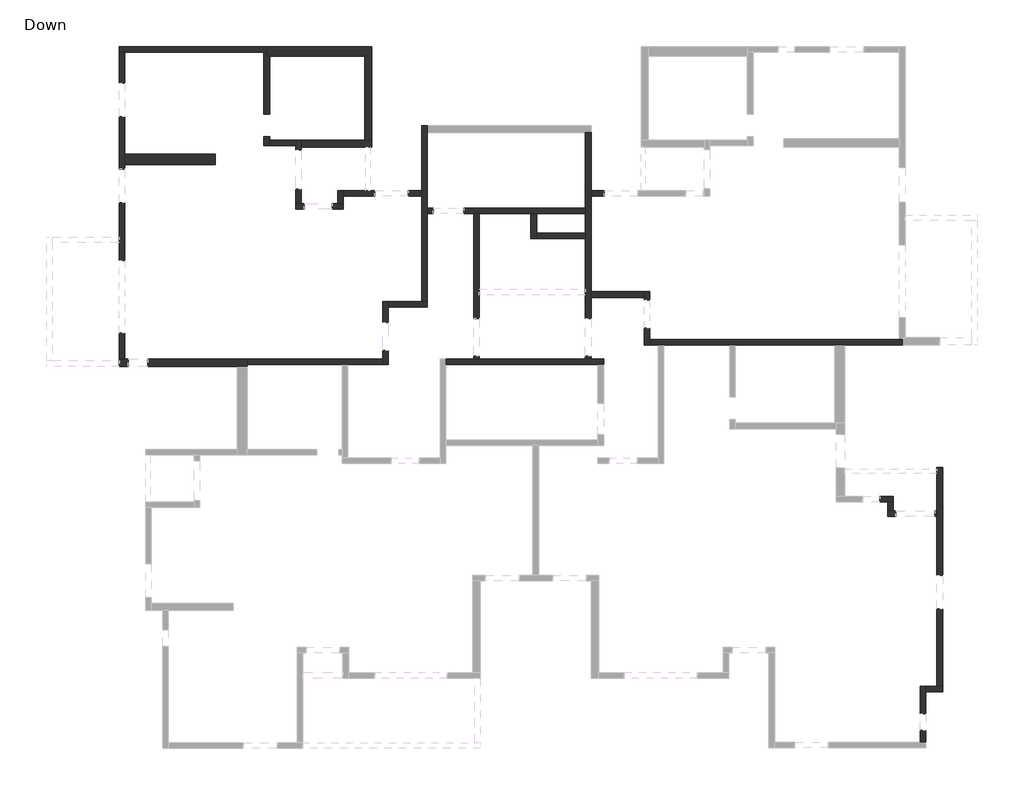
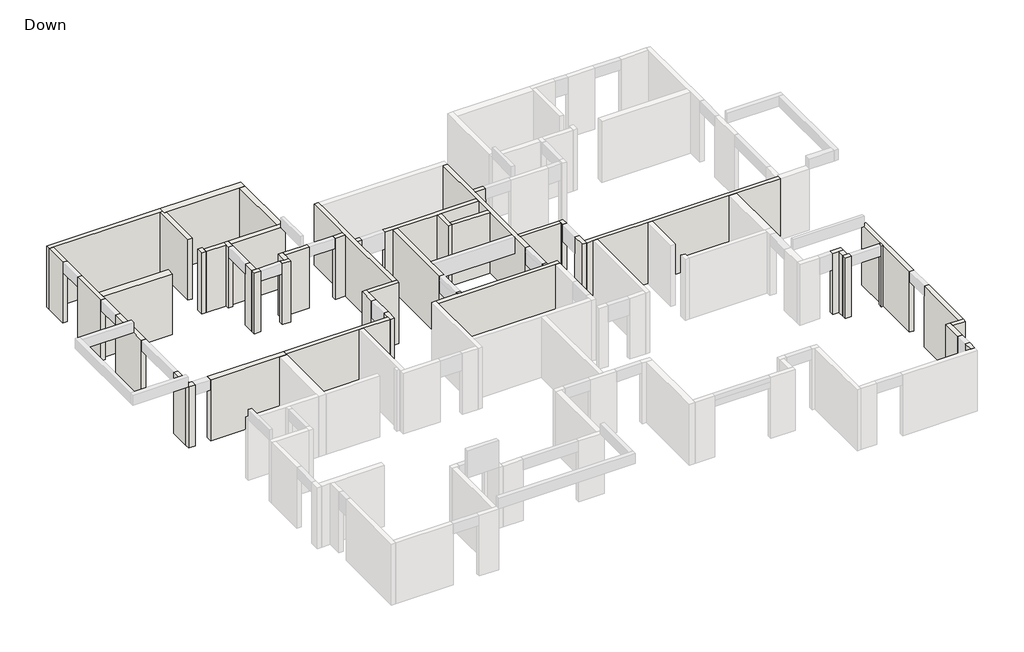
# One storey, part 2 of 3: 49 walls.
"""IFC4 building model written with IfcOpenShell, lengths in millimetres."""

from ifc_helpers import new_model, si_unit, origin, origin_with_axes, place, context, project, spatial, polyline, outline, extrude, faceted_brep, element, save

model = new_model("IFC4")

# Units and contexts
model_context = context("Model", 3, world=origin())
ifc_project = project(units=[si_unit("LENGTHUNIT", "METRE", prefix="MILLI")], contexts=[model_context])

# Site, building, storey
site = spatial("IfcSite", under=ifc_project)
building = spatial("IfcBuilding", under=site)
storey = spatial("IfcBuildingStorey", under=building, Name="Down", Elevation=0.0)

# Walls
placement = place(None, origin())
element("IfcWall", 1, ObjectType="20", at=placement, inside=storey, context=model_context, shape_type="Brep", body=[
    faceted_brep([(-5039.8370837, 11436.5624033, 0.0), (-10319.6462524, 11436.5624033, 0.0), (-10319.6462524, 11436.5624033, 3000.0), (-5039.8370837, 11436.5624033, 3000.0), (-5039.8370837, 11236.5624033, 0.0), (-5039.8370837, 11236.5624033, 3000.0), (-5139.8370837, 11236.5624033, 3000.0), (-10119.6462524, 11236.5624033, 3000.0), (-10319.6462524, 11236.5624033, 3000.0), (-10319.6462524, 11236.5624033, 0.0), (-10119.6462524, 11236.5624033, 0.0), (-5139.8370837, 11236.5624033, 0.0)], [[[0, 1, 2, 3]], [[4, 5, 6, 7, 8, 9, 10, 11]], [[1, 0, 4, 11, 10, 9]], [[3, 2, 8, 7, 6, 5]], [[0, 3, 5, 4]], [[2, 1, 9, 8]]]),
])
element("IfcWall", 2, ObjectType="20", at=placement, inside=storey, context=model_context, shape_type="Brep", body=[
    faceted_brep([(-10319.6462524, 11236.5624033, 0.0), (-10319.6462524, 10130.5632806, 0.0), (-10319.6462524, 10130.5632806, 2500.0), (-10319.6462524, 10130.5632806, 3000.0), (-10319.6462524, 11236.5624033, 3000.0), (-10119.6462524, 11236.5624033, 0.0), (-10119.6462524, 11236.5624033, 2780.0), (-10119.6462524, 11236.5624033, 3000.0), (-10119.6462524, 10130.5632806, 3000.0), (-10119.6462524, 10130.5632806, 2500.0), (-10119.6462524, 10130.5632806, 0.0)], [[[0, 1, 2, 3, 4]], [[5, 6, 7, 8, 9, 10]], [[1, 0, 5, 10]], [[3, 2, 1, 10, 9, 8]], [[4, 3, 8, 7]], [[0, 4, 7, 6, 5]]]),
])
element("IfcWall", 3, ObjectType="20", at=placement, inside=storey, context=model_context, shape_type="Brep", body=[
    faceted_brep([(-10319.6462524, 8930.3987709, 0.0), (-10319.6462524, 7055.0094311, 0.0), (-10319.6462524, 7055.0094311, 2500.0), (-10319.6462524, 7055.0094311, 3000.0), (-10319.6462524, 8930.3987709, 3000.0), (-10319.6462524, 8930.3987709, 2500.0), (-10119.6462524, 8930.3987709, 0.0), (-10119.6462524, 8930.3987709, 2500.0), (-10119.6462524, 8930.3987709, 3000.0), (-10119.6462524, 7575.1187953, 3000.0), (-10119.6462524, 7215.1187953, 3000.0), (-10119.6462524, 7055.0094311, 3000.0), (-10119.6462524, 7055.0094311, 2500.0), (-10119.6462524, 7055.0094311, 0.0), (-10119.6462524, 7215.1187953, 0.0), (-10119.6462524, 7575.1187953, 0.0)], [[[0, 1, 2, 3, 4, 5]], [[6, 7, 8, 9, 10, 11, 12, 13, 14, 15]], [[1, 0, 6, 15, 14, 13]], [[3, 2, 1, 13, 12, 11]], [[4, 3, 11, 10, 9, 8]], [[0, 5, 4, 8, 7, 6]]]),
])
element("IfcWall", 4, ObjectType="20", at=placement, inside=storey, context=model_context, shape_type="Brep", body=[
    faceted_brep([(-10319.6462524, 5854.8449214, 0.0), (-10319.6462524, 3780.4865094, 0.0), (-10319.6462524, 3780.4865094, 2500.0), (-10319.6462524, 3780.4865094, 3000.0), (-10319.6462524, 4616.1884177, 3000.0), (-10319.6462524, 5854.8449214, 3000.0), (-10319.6462524, 5854.8449214, 2500.0), (-10119.6462524, 5854.8449214, 0.0), (-10119.6462524, 5854.8449214, 2500.0), (-10119.6462524, 5854.8449214, 3000.0), (-10119.6462524, 3780.4865094, 3000.0), (-10119.6462524, 3780.4865094, 2500.0), (-10119.6462524, 3780.4865094, 0.0)], [[[0, 1, 2, 3, 4, 5, 6]], [[7, 8, 9, 10, 11, 12]], [[1, 0, 7, 12]], [[3, 2, 1, 12, 11, 10]], [[5, 4, 3, 10, 9]], [[0, 6, 5, 9, 8, 7]]]),
])
element("IfcWall", 5, ObjectType="20", at=placement, inside=storey, context=model_context, shape_type="Brep", body=[
    faceted_brep([(-10319.6462524, 1181.1884177, 0.0), (-10319.6462524, 251.1884177, 0.0), (-10319.6462524, 251.1884177, 3000.0), (-10319.6462524, 1181.1884177, 3000.0), (-10319.6462524, 1181.1884177, 2500.0), (-10119.6462524, 1181.1884177, 0.0), (-10119.6462524, 1181.1884177, 2500.0), (-10119.6462524, 1181.1884177, 3000.0), (-10119.6462524, 251.1884177, 3000.0), (-10119.6462524, 251.1884177, 2780.0), (-10119.6462524, 251.1884177, 0.0)], [[[0, 1, 2, 3, 4]], [[5, 6, 7, 8, 9, 10]], [[1, 0, 5, 10]], [[3, 2, 8, 7]], [[0, 4, 3, 7, 6, 5]], [[2, 1, 10, 9, 8]]]),
])
element("IfcWall", 6, ObjectType="20", at=placement, inside=storey, context=model_context, shape_type="Brep", body=[
    faceted_brep([(-5740.9338154, 51.1884177, 0.0), (-2336.5139865, 51.1884177, 0.0), (-2136.5139865, 51.1884177, 0.0), (-890.8131749, 51.1884177, 0.0), (-890.8131749, 51.1884177, 3000.0), (-2136.5139865, 51.1884177, 3000.0), (-2336.5139865, 51.1884177, 3000.0), (-5740.9338154, 51.1884177, 3000.0), (-5740.9338154, 51.1884177, 2780.0), (-5740.9338154, 251.1884177, 0.0), (-5740.9338154, 251.1884177, 3000.0), (-890.8131749, 251.1884177, 3000.0), (-890.8131749, 251.1884177, 2780.0), (-890.8131749, 251.1884177, 0.0)], [[[0, 1, 2, 3, 4, 5, 6, 7, 8]], [[9, 10, 11, 12, 13]], [[3, 2, 1, 0, 9, 13]], [[7, 6, 5, 4, 11, 10]], [[0, 8, 7, 10, 9]], [[4, 3, 13, 12, 11]]]),
])
element("IfcWall", 7, ObjectType="20", at=placement, inside=storey, context=model_context, shape_type="Brep", body=[
    faceted_brep([(-690.8131749, 51.1884177, 0.0), (-690.8131749, 556.7642019, 0.0), (-690.8131749, 556.7642019, 2180.0), (-690.8131749, 556.7642019, 3000.0), (-690.8131749, 51.1884177, 3000.0), (-690.8131749, 51.1884177, 2780.0), (-890.8131749, 51.1884177, 0.0), (-890.8131749, 51.1884177, 3000.0), (-890.8131749, 251.1884177, 3000.0), (-890.8131749, 556.7642019, 3000.0), (-890.8131749, 556.7642019, 2180.0), (-890.8131749, 556.7642019, 0.0), (-890.8131749, 251.1884177, 0.0)], [[[0, 1, 2, 3, 4, 5]], [[6, 7, 8, 9, 10, 11, 12]], [[1, 0, 6, 12, 11]], [[3, 2, 1, 11, 10, 9]], [[4, 3, 9, 8, 7]], [[0, 5, 4, 7, 6]]]),
])
element("IfcWall", 8, ObjectType="20", at=placement, inside=storey, context=model_context, shape_type="Brep", body=[
    faceted_brep([(-690.8131749, 1555.8429472, 0.0), (-690.8131749, 2105.1520062, 0.0), (-690.8131749, 2305.1520062, 0.0), (-690.8131749, 2305.1520062, 3000.0), (-690.8131749, 2105.1520062, 3000.0), (-690.8131749, 1555.8429472, 3000.0), (-690.8131749, 1555.8429472, 2180.0), (-890.8131749, 1555.8429472, 0.0), (-890.8131749, 1555.8429472, 2180.0), (-890.8131749, 1555.8429472, 3000.0), (-890.8131749, 2305.1520062, 3000.0), (-890.8131749, 2305.1520062, 2780.0), (-890.8131749, 2305.1520062, 0.0)], [[[0, 1, 2, 3, 4, 5, 6]], [[7, 8, 9, 10, 11, 12]], [[2, 1, 0, 7, 12]], [[5, 4, 3, 10, 9]], [[0, 6, 5, 9, 8, 7]], [[3, 2, 12, 11, 10]]]),
])
element("IfcWall", 9, ObjectType="20", at=placement, inside=storey, context=model_context, shape_type="Brep", body=[
    faceted_brep([(-690.8131749, 2105.1520062, 0.0), (708.320407, 2105.1520062, 0.0), (708.320407, 2105.1520062, 2780.0), (708.320407, 2105.1520062, 3000.0), (-690.8131749, 2105.1520062, 3000.0), (-690.8131749, 2105.1520062, 2780.0), (-690.8131749, 2305.1520062, 0.0), (-690.8131749, 2305.1520062, 3000.0), (508.320407, 2305.1520062, 3000.0), (708.320407, 2305.1520062, 3000.0), (708.320407, 2305.1520062, 0.0), (508.320407, 2305.1520062, 0.0)], [[[0, 1, 2, 3, 4, 5]], [[6, 7, 8, 9, 10, 11]], [[1, 0, 6, 11, 10]], [[4, 3, 9, 8, 7]], [[0, 5, 4, 7, 6]], [[3, 2, 1, 10, 9]]]),
])
element("IfcWall", 10, ObjectType="20", at=placement, inside=storey, context=model_context, shape_type="Brep", body=[
    faceted_brep([(708.320407, 2305.1520062, 0.0), (708.320407, 5455.8758492, 0.0), (708.320407, 5655.8758492, 0.0), (708.320407, 8355.1520062, 0.0), (708.320407, 8605.1520062, 0.0), (708.320407, 8605.1520062, 3000.0), (708.320407, 8355.1520062, 3000.0), (708.320407, 5655.8758492, 3000.0), (708.320407, 5455.8758492, 3000.0), (708.320407, 2305.1520062, 3000.0), (508.320407, 2305.1520062, 0.0), (508.320407, 2305.1520062, 2780.0), (508.320407, 2305.1520062, 3000.0), (508.320407, 6080.1520062, 3000.0), (508.320407, 6280.1520062, 3000.0), (508.320407, 8605.1520062, 3000.0), (508.320407, 8605.1520062, 0.0), (508.320407, 6280.1520062, 0.0), (508.320407, 6080.1520062, 0.0)], [[[0, 1, 2, 3, 4, 5, 6, 7, 8, 9]], [[10, 11, 12, 13, 14, 15, 16, 17, 18]], [[4, 3, 2, 1, 0, 10, 18, 17, 16]], [[9, 8, 7, 6, 5, 15, 14, 13, 12]], [[0, 9, 12, 11, 10]], [[5, 4, 16, 15]]]),
])
element("IfcWall", 11, ObjectType="20", at=placement, inside=storey, context=model_context, shape_type="Brep", body=[
    faceted_brep([(708.320407, 5455.8758492, 0.0), (909.4061714, 5455.8758492, 0.0), (909.4061714, 5455.8758492, 2180.0), (909.4061714, 5455.8758492, 3000.0), (708.320407, 5455.8758492, 3000.0), (708.320407, 5455.8758492, 2780.0), (708.320407, 5655.8758492, 0.0), (708.320407, 5655.8758492, 2780.0), (708.320407, 5655.8758492, 3000.0), (909.4061714, 5655.8758492, 3000.0), (909.4061714, 5655.8758492, 2180.0), (909.4061714, 5655.8758492, 0.0)], [[[0, 1, 2, 3, 4, 5]], [[6, 7, 8, 9, 10, 11]], [[1, 0, 6, 11]], [[3, 2, 1, 11, 10, 9]], [[4, 3, 9, 8]], [[0, 5, 4, 8, 7, 6]]]),
])
element("IfcWall", 12, ObjectType="20", at=placement, inside=storey, context=model_context, shape_type="Brep", body=[
    faceted_brep([(508.320407, 6280.1520062, 0.0), (28.320407, 6280.1520062, 0.0), (28.320407, 6280.1520062, 2500.0), (28.320407, 6280.1520062, 3000.0), (508.320407, 6280.1520062, 3000.0), (508.320407, 6080.1520062, 0.0), (508.320407, 6080.1520062, 2780.0), (508.320407, 6080.1520062, 3000.0), (28.320407, 6080.1520062, 3000.0), (28.320407, 6080.1520062, 2500.0), (28.320407, 6080.1520062, 0.0)], [[[0, 1, 2, 3, 4]], [[5, 6, 7, 8, 9, 10]], [[1, 0, 5, 10]], [[3, 2, 1, 10, 9, 8]], [[4, 3, 8, 7]], [[0, 4, 7, 6, 5]]]),
])
element("IfcWall", 13, ObjectType="20", at=placement, inside=storey, context=model_context, shape_type="Brep", body=[
    faceted_brep([(-1171.679593, 6280.1520062, 0.0), (-2301.679593, 6280.1520062, 0.0), (-2301.679593, 6280.1520062, 3000.0), (-1339.8370837, 6280.1520062, 3000.0), (-1171.679593, 6280.1520062, 3000.0), (-1171.679593, 6280.1520062, 2500.0), (-1171.679593, 6080.1520062, 0.0), (-1171.679593, 6080.1520062, 2500.0), (-1171.679593, 6080.1520062, 3000.0), (-2301.679593, 6080.1520062, 3000.0), (-2301.679593, 6080.1520062, 2780.0), (-2301.679593, 6080.1520062, 0.0)], [[[0, 1, 2, 3, 4, 5]], [[6, 7, 8, 9, 10, 11]], [[1, 0, 6, 11]], [[4, 3, 2, 9, 8]], [[0, 5, 4, 8, 7, 6]], [[2, 1, 11, 10, 9]]]),
])
element("IfcWall", 14, ObjectType="20", at=placement, inside=storey, context=model_context, shape_type="Brep", body=[
    faceted_brep([(-2501.679593, 6280.1520062, 0.0), (-2501.679593, 5815.1520062, 0.0), (-2501.679593, 5815.1520062, 2780.0), (-2501.679593, 5815.1520062, 3000.0), (-2501.679593, 6280.1520062, 3000.0), (-2501.679593, 6280.1520062, 2780.0), (-2301.679593, 6280.1520062, 0.0), (-2301.679593, 6280.1520062, 3000.0), (-2301.679593, 6080.1520062, 3000.0), (-2301.679593, 5815.1520062, 3000.0), (-2301.679593, 5815.1520062, 0.0), (-2301.679593, 6080.1520062, 0.0)], [[[0, 1, 2, 3, 4, 5]], [[6, 7, 8, 9, 10, 11]], [[1, 0, 6, 11, 10]], [[4, 3, 9, 8, 7]], [[0, 5, 4, 7, 6]], [[3, 2, 1, 10, 9]]]),
])
element("IfcWall", 15, ObjectType="20", at=placement, inside=storey, context=model_context, shape_type="Brep", body=[
    faceted_brep([(-2301.679593, 5815.1520062, 0.0), (-2501.679593, 5815.1520062, 0.0), (-2696.679593, 5815.1520062, 0.0), (-2696.679593, 5815.1520062, 2500.0), (-2696.679593, 5815.1520062, 3000.0), (-2501.679593, 5815.1520062, 3000.0), (-2301.679593, 5815.1520062, 3000.0), (-2301.679593, 5615.1520062, 0.0), (-2301.679593, 5615.1520062, 2780.0), (-2301.679593, 5615.1520062, 3000.0), (-2696.679593, 5615.1520062, 3000.0), (-2696.679593, 5615.1520062, 2500.0), (-2696.679593, 5615.1520062, 0.0)], [[[0, 1, 2, 3, 4, 5, 6]], [[7, 8, 9, 10, 11, 12]], [[2, 1, 0, 7, 12]], [[4, 3, 2, 12, 11, 10]], [[6, 5, 4, 10, 9]], [[0, 6, 9, 8, 7]]]),
])
element("IfcWall", 16, ObjectType="20", at=placement, inside=storey, context=model_context, shape_type="Brep", body=[
    faceted_brep([(-3696.679593, 5815.1520062, 0.0), (-3799.8370837, 5815.1520062, 0.0), (-3999.8370837, 5815.1520062, 0.0), (-3999.8370837, 5815.1520062, 3000.0), (-3799.8370837, 5815.1520062, 3000.0), (-3696.679593, 5815.1520062, 3000.0), (-3696.679593, 5815.1520062, 2500.0), (-3696.679593, 5615.1520062, 0.0), (-3696.679593, 5615.1520062, 2500.0), (-3696.679593, 5615.1520062, 3000.0), (-3999.8370837, 5615.1520062, 3000.0), (-3999.8370837, 5615.1520062, 2780.0), (-3999.8370837, 5615.1520062, 0.0)], [[[0, 1, 2, 3, 4, 5, 6]], [[7, 8, 9, 10, 11, 12]], [[2, 1, 0, 7, 12]], [[5, 4, 3, 10, 9]], [[0, 6, 5, 9, 8, 7]], [[3, 2, 12, 11, 10]]]),
])
element("IfcWall", 17, ObjectType="20", at=placement, inside=storey, context=model_context, shape_type="Brep", body=[
    faceted_brep([(-3799.8370837, 5815.1520062, 0.0), (-3799.8370837, 6335.1520062, 0.0), (-3799.8370837, 6335.1520062, 2500.0), (-3799.8370837, 6335.1520062, 3000.0), (-3799.8370837, 5815.1520062, 3000.0), (-3799.8370837, 5815.1520062, 2780.0), (-3999.8370837, 5815.1520062, 0.0), (-3999.8370837, 5815.1520062, 3000.0), (-3999.8370837, 6335.1520062, 3000.0), (-3999.8370837, 6335.1520062, 2500.0), (-3999.8370837, 6335.1520062, 0.0)], [[[0, 1, 2, 3, 4, 5]], [[6, 7, 8, 9, 10]], [[1, 0, 6, 10]], [[3, 2, 1, 10, 9, 8]], [[4, 3, 8, 7]], [[0, 5, 4, 7, 6]]]),
])
element("IfcWall", 18, ObjectType="20", at=placement, inside=storey, context=model_context, shape_type="Brep", body=[
    faceted_brep([(-5139.8370837, 11236.5624033, 0.0), (-5139.8370837, 9006.5624033, 0.0), (-5139.8370837, 9006.5624033, 2780.0), (-5139.8370837, 9006.5624033, 3000.0), (-5139.8370837, 11236.5624033, 3000.0), (-5139.8370837, 11236.5624033, 2780.0), (-4939.8370837, 11086.5624033, 0.0), (-4939.8370837, 11086.5624033, 2780.0), (-4939.8370837, 11086.5624033, 3000.0), (-4939.8370837, 9006.5624033, 3000.0), (-4939.8370837, 9006.5624033, 2780.0), (-4939.8370837, 9006.5624033, 0.0), (-5039.8370837, 11236.5624033, 0.0), (-5039.8370837, 11086.5624033, 0.0), (-5039.8370837, 11086.5624033, 3000.0), (-5039.8370837, 11236.5624033, 3000.0)], [[[0, 1, 2, 3, 4, 5]], [[6, 7, 8, 9, 10, 11]], [[1, 0, 12, 13, 6, 11]], [[3, 2, 1, 11, 10, 9]], [[4, 3, 9, 8, 14, 15]], [[0, 5, 4, 15, 12]], [[15, 14, 13, 12]], [[14, 8, 7, 6, 13]]]),
])
element("IfcWall", 19, ObjectType="20", at=placement, inside=storey, context=model_context, shape_type="Brep", body=[
    faceted_brep([(-5139.8370837, 8206.5624033, 0.0), (-5139.8370837, 7886.5624033, 0.0), (-5139.8370837, 7886.5624033, 2780.0), (-5139.8370837, 7886.5624033, 3000.0), (-5139.8370837, 8206.5624033, 3000.0), (-5139.8370837, 8206.5624033, 2780.0), (-4939.8370837, 8206.5624033, 0.0), (-4939.8370837, 8206.5624033, 2780.0), (-4939.8370837, 8206.5624033, 3000.0), (-4939.8370837, 8086.5624033, 3000.0), (-4939.8370837, 7886.5624033, 3000.0), (-4939.8370837, 7886.5624033, 0.0), (-4939.8370837, 8086.5624033, 0.0)], [[[0, 1, 2, 3, 4, 5]], [[6, 7, 8, 9, 10, 11, 12]], [[1, 0, 6, 12, 11]], [[4, 3, 10, 9, 8]], [[0, 5, 4, 8, 7, 6]], [[3, 2, 1, 11, 10]]]),
])
element("IfcWall", 20, ObjectType="20", at=placement, inside=storey, context=model_context, shape_type="Brep", body=[
    faceted_brep([(-4939.8370837, 7886.5624033, 0.0), (-3999.8370837, 7886.5624033, 0.0), (-3999.8370837, 7886.5624033, 2780.0), (-3999.8370837, 7886.5624033, 3000.0), (-4939.8370837, 7886.5624033, 3000.0), (-4939.8370837, 8086.5624033, 0.0), (-4939.8370837, 8086.5624033, 2780.0), (-4939.8370837, 8086.5624033, 3000.0), (-3999.8370837, 8086.5624033, 3000.0), (-3999.8370837, 8086.5624033, 0.0)], [[[0, 1, 2, 3, 4]], [[5, 6, 7, 8, 9]], [[1, 0, 5, 9]], [[4, 3, 8, 7]], [[0, 4, 7, 6, 5]], [[3, 2, 1, 9, 8]]]),
])
element("IfcWall", 21, ObjectType="20", at=placement, inside=storey, context=model_context, shape_type="Brep", body=[
    faceted_brep([(-3999.8370837, 8086.5624033, 0.0), (-3999.8370837, 7886.5624033, 0.0), (-3999.8370837, 7726.5624033, 0.0), (-3999.8370837, 7726.5624033, 2500.0), (-3999.8370837, 7726.5624033, 3000.0), (-3999.8370837, 7886.5624033, 3000.0), (-3999.8370837, 8086.5624033, 3000.0), (-3799.8370837, 8086.5624033, 0.0), (-3799.8370837, 8086.5624033, 3000.0), (-3799.8370837, 7836.5624033, 3000.0), (-3799.8370837, 7726.5624033, 3000.0), (-3799.8370837, 7726.5624033, 2500.0), (-3799.8370837, 7726.5624033, 0.0), (-3799.8370837, 7836.5624033, 0.0)], [[[0, 1, 2, 3, 4, 5, 6]], [[7, 8, 9, 10, 11, 12, 13]], [[2, 1, 0, 7, 13, 12]], [[4, 3, 2, 12, 11, 10]], [[6, 5, 4, 10, 9, 8]], [[0, 6, 8, 7]]]),
])
element("IfcWall", 22, ObjectType="20", at=placement, inside=storey, context=model_context, shape_type="Brep", body=[
    faceted_brep([(6363.320407, 8355.1520062, 0.0), (6363.320407, 5655.8758492, 0.0), (6363.320407, 5455.8758492, 0.0), (6363.320407, 4755.8758492, 0.0), (6363.320407, 4555.8758492, 0.0), (6363.320407, 1705.1520062, 0.0), (6363.320407, 1705.1520062, 2180.0), (6363.320407, 1705.1520062, 2780.0), (6363.320407, 1705.1520062, 3000.0), (6363.320407, 2545.8758492, 3000.0), (6363.320407, 2745.8758492, 3000.0), (6363.320407, 4555.8758492, 3000.0), (6363.320407, 4755.8758492, 3000.0), (6363.320407, 5455.8758492, 3000.0), (6363.320407, 5655.8758492, 3000.0), (6363.320407, 8355.1520062, 3000.0), (6563.320407, 8355.1520062, 0.0), (6563.320407, 8355.1520062, 3000.0), (6563.320407, 6284.3445962, 3000.0), (6563.320407, 6084.3445962, 3000.0), (6563.320407, 2655.1520062, 3000.0), (6563.320407, 2455.1520062, 3000.0), (6563.320407, 1705.1520062, 3000.0), (6563.320407, 1705.1520062, 2180.0), (6563.320407, 1705.1520062, 0.0), (6563.320407, 2455.1520062, 0.0), (6563.320407, 2655.1520062, 0.0), (6563.320407, 6084.3445962, 0.0), (6563.320407, 6284.3445962, 0.0), (6368.320407, 1705.1520062, 3000.0)], [[[0, 1, 2, 3, 4, 5, 6, 7, 8, 9, 10, 11, 12, 13, 14, 15]], [[16, 17, 18, 19, 20, 21, 22, 23, 24, 25, 26, 27, 28]], [[5, 4, 3, 2, 1, 0, 16, 28, 27, 26, 25, 24]], [[8, 7, 6, 5, 24, 23, 22, 29]], [[15, 14, 13, 12, 11, 10, 9, 8, 29, 22, 21, 20, 19, 18, 17]], [[0, 15, 17, 16]]]),
])
element("IfcWall", 23, ObjectType="20", at=placement, inside=storey, context=model_context, shape_type="Brep", body=[
    faceted_brep([(6563.320407, 2455.1520062, 0.0), (8463.320407, 2455.1520062, 0.0), (8463.320407, 2455.1520062, 2780.0), (8463.320407, 2455.1520062, 3000.0), (6563.320407, 2455.1520062, 3000.0), (6563.320407, 2455.1520062, 2780.0), (6563.320407, 2655.1520062, 0.0), (6563.320407, 2655.1520062, 2780.0), (6563.320407, 2655.1520062, 3000.0), (8463.320407, 2655.1520062, 3000.0), (8463.320407, 2655.1520062, 0.0)], [[[0, 1, 2, 3, 4, 5]], [[6, 7, 8, 9, 10]], [[1, 0, 6, 10]], [[4, 3, 9, 8]], [[0, 5, 4, 8, 7, 6]], [[3, 2, 1, 10, 9]]]),
])
element("IfcWall", 24, ObjectType="20", at=placement, inside=storey, context=model_context, shape_type="Brep", body=[
    faceted_brep([(8463.320407, 2655.1520062, 0.0), (8463.320407, 2455.1520062, 0.0), (8463.320407, 2355.1520062, 0.0), (8463.320407, 2355.1520062, 2180.0), (8463.320407, 2355.1520062, 3000.0), (8463.320407, 2455.1520062, 3000.0), (8463.320407, 2655.1520062, 3000.0), (8663.320407, 2655.1520062, 0.0), (8663.320407, 2655.1520062, 2780.0), (8663.320407, 2655.1520062, 3000.0), (8663.320407, 2355.1520062, 3000.0), (8663.320407, 2355.1520062, 2180.0), (8663.320407, 2355.1520062, 0.0)], [[[0, 1, 2, 3, 4, 5, 6]], [[7, 8, 9, 10, 11, 12]], [[2, 1, 0, 7, 12]], [[4, 3, 2, 12, 11, 10]], [[6, 5, 4, 10, 9]], [[0, 6, 9, 8, 7]]]),
])
element("IfcWall", 25, ObjectType="20", at=placement, inside=storey, context=model_context, shape_type="Brep", body=[
    faceted_brep([(6363.320407, 5655.8758492, 0.0), (2013.320407, 5655.8758492, 0.0), (2013.320407, 5655.8758492, 2180.0), (2013.320407, 5655.8758492, 3000.0), (2460.820407, 5655.8758492, 3000.0), (6363.320407, 5655.8758492, 3000.0), (6363.320407, 5455.8758492, 0.0), (6363.320407, 5455.8758492, 3000.0), (4613.320407, 5455.8758492, 3000.0), (4413.320407, 5455.8758492, 3000.0), (2560.820407, 5455.8758492, 3000.0), (2360.820407, 5455.8758492, 3000.0), (2013.320407, 5455.8758492, 3000.0), (2013.320407, 5455.8758492, 2180.0), (2013.320407, 5455.8758492, 0.0), (2360.820407, 5455.8758492, 0.0), (2560.820407, 5455.8758492, 0.0), (4413.320407, 5455.8758492, 0.0), (4613.320407, 5455.8758492, 0.0)], [[[0, 1, 2, 3, 4, 5]], [[6, 7, 8, 9, 10, 11, 12, 13, 14, 15, 16, 17, 18]], [[1, 0, 6, 18, 17, 16, 15, 14]], [[3, 2, 1, 14, 13, 12]], [[5, 4, 3, 12, 11, 10, 9, 8, 7]], [[0, 5, 7, 6]]]),
])
element("IfcWall", 26, ObjectType="20", at=placement, inside=storey, context=model_context, shape_type="Brep", body=[
    faceted_brep([(2360.820407, 5455.8758492, 0.0), (2360.820407, 1705.8758492, 0.0), (2360.820407, 1705.8758492, 2180.0), (2360.820407, 1705.8758492, 2780.0), (2360.820407, 1705.8758492, 3000.0), (2360.820407, 5455.8758492, 3000.0), (2360.820407, 5455.8758492, 2780.0), (2560.820407, 5455.8758492, 0.0), (2560.820407, 5455.8758492, 3000.0), (2560.820407, 2745.8758492, 3000.0), (2560.820407, 2545.8758492, 3000.0), (2560.820407, 1705.8758492, 3000.0), (2560.820407, 1705.8758492, 2180.0), (2560.820407, 1705.8758492, 0.0), (2363.3932055, 1705.8758492, 3000.0)], [[[0, 1, 2, 3, 4, 5, 6]], [[7, 8, 9, 10, 11, 12, 13]], [[1, 0, 7, 13]], [[4, 3, 2, 1, 13, 12, 11, 14]], [[5, 4, 14, 11, 10, 9, 8]], [[0, 6, 5, 8, 7]]]),
])
element("IfcWall", 27, ObjectType="20", at=placement, inside=storey, context=model_context, shape_type="Brep", body=[
    faceted_brep([(2360.820407, 352.3535615, 0.0), (2360.820407, 252.3535615, 0.0), (2360.820407, 252.3535615, 2780.0), (2360.820407, 252.3535615, 3000.0), (2360.820407, 352.3535615, 3000.0), (2360.820407, 352.3535615, 2780.0), (2360.820407, 352.3535615, 2180.0), (2560.820407, 352.3535615, 0.0), (2560.820407, 352.3535615, 2180.0), (2560.820407, 352.3535615, 3000.0), (2560.820407, 252.3535615, 3000.0), (2560.820407, 252.3535615, 0.0), (2363.3932055, 352.3535615, 3000.0)], [[[0, 1, 2, 3, 4, 5, 6]], [[7, 8, 9, 10, 11]], [[1, 0, 7, 11]], [[4, 3, 10, 9, 12]], [[0, 6, 5, 4, 12, 9, 8, 7]], [[3, 2, 1, 11, 10]]]),
])
element("IfcWall", 28, ObjectType="20", at=placement, inside=storey, context=model_context, shape_type="Brep", body=[
    faceted_brep([(1360.820407, 52.3535615, 0.0), (6810.820407, 52.3535615, 0.0), (7010.820407, 52.3535615, 0.0), (7010.820407, 52.3535615, 3000.0), (6810.820407, 52.3535615, 3000.0), (1360.820407, 52.3535615, 3000.0), (1360.820407, 252.3535615, 0.0), (1360.820407, 252.3535615, 3000.0), (2360.820407, 252.3535615, 3000.0), (2560.820407, 252.3535615, 3000.0), (6363.320407, 252.3535615, 3000.0), (6563.320407, 252.3535615, 3000.0), (7010.820407, 252.3535615, 3000.0), (7010.820407, 252.3535615, 2780.0), (7010.820407, 252.3535615, 0.0), (6563.320407, 252.3535615, 0.0), (6363.320407, 252.3535615, 0.0), (2560.820407, 252.3535615, 0.0), (2360.820407, 252.3535615, 0.0)], [[[0, 1, 2, 3, 4, 5]], [[6, 7, 8, 9, 10, 11, 12, 13, 14, 15, 16, 17, 18]], [[2, 1, 0, 6, 18, 17, 16, 15, 14]], [[5, 4, 3, 12, 11, 10, 9, 8, 7]], [[3, 2, 14, 13, 12]], [[0, 5, 7, 6]]]),
])
element("IfcWall", 29, ObjectType="20", at=placement, inside=storey, context=model_context, shape_type="Brep", body=[
    faceted_brep([(18537.905294, -13477.9835498, 0.0), (18537.905294, -13047.9835498, 0.0), (18537.905294, -13047.9835498, 2180.0), (18537.905294, -13047.9835498, 3000.0), (18537.905294, -13477.9835498, 3000.0), (18337.905294, -13477.9835498, 0.0), (18337.905294, -13477.9835498, 2780.0), (18337.905294, -13477.9835498, 3000.0), (18337.905294, -13047.9835498, 3000.0), (18337.905294, -13047.9835498, 2180.0), (18337.905294, -13047.9835498, 0.0)], [[[0, 1, 2, 3, 4]], [[5, 6, 7, 8, 9, 10]], [[1, 0, 5, 10]], [[3, 2, 1, 10, 9, 8]], [[4, 3, 8, 7]], [[0, 4, 7, 6, 5]]]),
])
element("IfcWall", 30, ObjectType="20", at=placement, inside=storey, context=model_context, shape_type="Brep", body=[
    faceted_brep([(18537.905294, -12447.9835498, 0.0), (18537.905294, -11672.9835498, 0.0), (18537.905294, -11472.9835498, 0.0), (18537.905294, -11472.9835498, 3000.0), (18537.905294, -11672.9835498, 3000.0), (18537.905294, -12447.9835498, 3000.0), (18537.905294, -12447.9835498, 2180.0), (18337.905294, -12447.9835498, 0.0), (18337.905294, -12447.9835498, 2180.0), (18337.905294, -12447.9835498, 3000.0), (18337.905294, -11472.9835498, 3000.0), (18337.905294, -11472.9835498, 2780.0), (18337.905294, -11472.9835498, 0.0)], [[[0, 1, 2, 3, 4, 5, 6]], [[7, 8, 9, 10, 11, 12]], [[2, 1, 0, 7, 12]], [[5, 4, 3, 10, 9]], [[0, 6, 5, 9, 8, 7]], [[3, 2, 12, 11, 10]]]),
])
element("IfcWall", 31, ObjectType="20", at=placement, inside=storey, context=model_context, shape_type="Brep", body=[
    faceted_brep([(18537.905294, -11672.9835498, 0.0), (19137.905294, -11672.9835498, 0.0), (19137.905294, -11672.9835498, 3000.0), (18537.905294, -11672.9835498, 3000.0), (18537.905294, -11472.9835498, 0.0), (18537.905294, -11472.9835498, 3000.0), (18937.905294, -11472.9835498, 3000.0), (19137.905294, -11472.9835498, 3000.0), (19137.905294, -11472.9835498, 0.0), (18937.905294, -11472.9835498, 0.0)], [[[0, 1, 2, 3]], [[4, 5, 6, 7, 8, 9]], [[1, 0, 4, 9, 8]], [[3, 2, 7, 6, 5]], [[0, 3, 5, 4]], [[2, 1, 8, 7]]]),
])
element("IfcWall", 32, ObjectType="20", at=placement, inside=storey, context=model_context, shape_type="Brep", body=[
    faceted_brep([(19137.905294, -11472.9835498, 0.0), (19137.905294, -8697.9835498, 0.0), (19137.905294, -8697.9835498, 2500.0), (19137.905294, -8697.9835498, 3000.0), (19137.905294, -11472.9835498, 3000.0), (18937.905294, -11472.9835498, 0.0), (18937.905294, -11472.9835498, 2780.0), (18937.905294, -11472.9835498, 3000.0), (18937.905294, -8697.9835498, 3000.0), (18937.905294, -8697.9835498, 2500.0), (18937.905294, -8697.9835498, 0.0)], [[[0, 1, 2, 3, 4]], [[5, 6, 7, 8, 9, 10]], [[1, 0, 5, 10]], [[3, 2, 1, 10, 9, 8]], [[4, 3, 8, 7]], [[0, 4, 7, 6, 5]]]),
])
element("IfcWall", 33, ObjectType="20", at=placement, inside=storey, context=model_context, shape_type="Brep", body=[
    faceted_brep([(19137.905294, -7497.9835498, 0.0), (19137.905294, -3642.9835498, 0.0), (19137.905294, -3642.9835498, 3000.0), (19137.905294, -7497.9835498, 3000.0), (19137.905294, -7497.9835498, 2500.0), (18937.905294, -7497.9835498, 0.0), (18937.905294, -7497.9835498, 2500.0), (18937.905294, -7497.9835498, 3000.0), (18937.905294, -5382.9835498, 3000.0), (18937.905294, -5182.9835498, 3000.0), (18937.905294, -3693.5538503, 3000.0), (18937.905294, -3642.9835498, 3000.0), (18937.905294, -3642.9835498, 0.0), (18937.905294, -5182.9835498, 0.0), (18937.905294, -5382.9835498, 0.0)], [[[0, 1, 2, 3, 4]], [[5, 6, 7, 8, 9, 10, 11, 12, 13, 14]], [[1, 0, 5, 14, 13, 12]], [[2, 1, 12, 11]], [[3, 2, 11, 10, 9, 8, 7]], [[0, 4, 3, 7, 6, 5]]]),
])
element("IfcWall", 34, ObjectType="20", at=placement, inside=storey, context=model_context, shape_type="Brep", body=[
    faceted_brep([(18937.905294, -5182.9835498, 0.0), (18857.905294, -5182.9835498, 0.0), (18857.905294, -5182.9835498, 2500.0), (18857.905294, -5182.9835498, 3000.0), (18937.905294, -5182.9835498, 3000.0), (18937.905294, -5182.9835498, 2780.0), (18937.905294, -5382.9835498, 0.0), (18937.905294, -5382.9835498, 2780.0), (18937.905294, -5382.9835498, 3000.0), (18857.905294, -5382.9835498, 3000.0), (18857.905294, -5382.9835498, 2500.0), (18857.905294, -5382.9835498, 0.0)], [[[0, 1, 2, 3, 4, 5]], [[6, 7, 8, 9, 10, 11]], [[1, 0, 6, 11]], [[3, 2, 1, 11, 10, 9]], [[4, 3, 9, 8]], [[0, 5, 4, 8, 7, 6]]]),
])
element("IfcWall", 35, ObjectType="20", at=placement, inside=storey, context=model_context, shape_type="Brep", body=[
    faceted_brep([(17457.905294, -5182.9835498, 0.0), (17377.905294, -5182.9835498, 0.0), (17177.905294, -5182.9835498, 0.0), (17177.905294, -5182.9835498, 3000.0), (17377.905294, -5182.9835498, 3000.0), (17457.905294, -5182.9835498, 3000.0), (17457.905294, -5182.9835498, 2500.0), (17457.905294, -5382.9835498, 0.0), (17457.905294, -5382.9835498, 2500.0), (17457.905294, -5382.9835498, 3000.0), (17177.905294, -5382.9835498, 3000.0), (17177.905294, -5382.9835498, 2780.0), (17177.905294, -5382.9835498, 0.0)], [[[0, 1, 2, 3, 4, 5, 6]], [[7, 8, 9, 10, 11, 12]], [[2, 1, 0, 7, 12]], [[5, 4, 3, 10, 9]], [[0, 6, 5, 9, 8, 7]], [[3, 2, 12, 11, 10]]]),
])
element("IfcWall", 36, ObjectType="20", at=placement, inside=storey, context=model_context, shape_type="Brep", body=[
    faceted_brep([(17377.905294, -5182.9835498, 0.0), (17377.905294, -4862.9835498, 0.0), (17377.905294, -4862.9835498, 3000.0), (17377.905294, -5182.9835498, 3000.0), (17377.905294, -5182.9835498, 2780.0), (17177.905294, -5182.9835498, 0.0), (17177.905294, -5182.9835498, 3000.0), (17177.905294, -4862.9835498, 3000.0), (17177.905294, -4862.9835498, 2780.0), (17177.905294, -4862.9835498, 0.0)], [[[0, 1, 2, 3, 4]], [[5, 6, 7, 8, 9]], [[1, 0, 5, 9]], [[3, 2, 7, 6]], [[0, 4, 3, 6, 5]], [[2, 1, 9, 8, 7]]]),
])
element("IfcWall", 37, ObjectType="20", at=placement, inside=storey, context=model_context, shape_type="Brep", body=[
    faceted_brep([(17377.905294, -4662.9835498, 0.0), (16897.905294, -4662.9835498, 0.0), (16897.905294, -4662.9835498, 2180.0), (16897.905294, -4662.9835498, 3000.0), (17377.905294, -4662.9835498, 3000.0), (17377.905294, -4662.9835498, 2780.0), (17377.905294, -4862.9835498, 0.0), (17377.905294, -4862.9835498, 3000.0), (17177.905294, -4862.9835498, 3000.0), (16897.905294, -4862.9835498, 3000.0), (16897.905294, -4862.9835498, 2180.0), (16897.905294, -4862.9835498, 0.0), (17177.905294, -4862.9835498, 0.0)], [[[0, 1, 2, 3, 4, 5]], [[6, 7, 8, 9, 10, 11, 12]], [[1, 0, 6, 12, 11]], [[3, 2, 1, 11, 10, 9]], [[4, 3, 9, 8, 7]], [[0, 5, 4, 7, 6]]]),
])
element("IfcWall", 38, ObjectType="20", at=placement, inside=storey, context=model_context, shape_type="Brep", body=[
    faceted_brep([(8663.320407, 752.0164502, 0.0), (8663.320407, 952.0164502, 0.0), (8663.320407, 1352.0164502, 0.0), (8663.320407, 1352.0164502, 2180.0), (8663.320407, 1352.0164502, 3000.0), (8663.320407, 952.0164502, 3000.0), (8663.320407, 752.0164502, 3000.0), (8463.320407, 752.0164502, 0.0), (8463.320407, 752.0164502, 2780.0), (8463.320407, 752.0164502, 3000.0), (8463.320407, 1352.0164502, 3000.0), (8463.320407, 1352.0164502, 2180.0), (8463.320407, 1352.0164502, 0.0)], [[[0, 1, 2, 3, 4, 5, 6]], [[7, 8, 9, 10, 11, 12]], [[2, 1, 0, 7, 12]], [[4, 3, 2, 12, 11, 10]], [[6, 5, 4, 10, 9]], [[0, 6, 9, 8, 7]]]),
])
element("IfcWall", 39, ObjectType="20", at=placement, inside=storey, context=model_context, shape_type="Brep", body=[
    faceted_brep([(8663.320407, 752.0164502, 0.0), (8963.320407, 752.0164502, 0.0), (9163.320407, 752.0164502, 0.0), (11517.905294, 752.0164502, 0.0), (11717.905294, 752.0164502, 0.0), (15289.9526685, 752.0164502, 0.0), (15639.9526685, 752.0164502, 0.0), (17697.905294, 752.0164502, 0.0), (17697.905294, 752.0164502, 3000.0), (15639.9526685, 752.0164502, 3000.0), (15289.9526685, 752.0164502, 3000.0), (11717.905294, 752.0164502, 3000.0), (11517.905294, 752.0164502, 3000.0), (9163.320407, 752.0164502, 3000.0), (8963.320407, 752.0164502, 3000.0), (8663.320407, 752.0164502, 3000.0), (8663.320407, 952.0164502, 0.0), (8663.320407, 952.0164502, 2780.0), (8663.320407, 952.0164502, 3000.0), (17597.905294, 952.0164502, 3000.0), (17697.905294, 952.0164502, 3000.0), (17697.905294, 952.0164502, 0.0), (17597.905294, 952.0164502, 0.0)], [[[0, 1, 2, 3, 4, 5, 6, 7, 8, 9, 10, 11, 12, 13, 14, 15]], [[16, 17, 18, 19, 20, 21, 22]], [[7, 6, 5, 4, 3, 2, 1, 0, 16, 22, 21]], [[8, 7, 21, 20]], [[15, 14, 13, 12, 11, 10, 9, 8, 20, 19, 18]], [[0, 15, 18, 17, 16]]]),
])
element("IfcWall", 40, ObjectType="20", at=placement, inside=storey, context=model_context, shape_type="Brep", body=[
    faceted_brep([(7043.320407, 6284.3445962, 0.0), (6563.320407, 6284.3445962, 0.0), (6563.320407, 6284.3445962, 3000.0), (7043.320407, 6284.3445962, 3000.0), (7043.320407, 6284.3445962, 2500.0), (7043.320407, 6084.3445962, 0.0), (7043.320407, 6084.3445962, 2500.0), (7043.320407, 6084.3445962, 3000.0), (6563.320407, 6084.3445962, 3000.0), (6563.320407, 6084.3445962, 2780.0), (6563.320407, 6084.3445962, 0.0)], [[[0, 1, 2, 3, 4]], [[5, 6, 7, 8, 9, 10]], [[1, 0, 5, 10]], [[3, 2, 8, 7]], [[0, 4, 3, 7, 6, 5]], [[2, 1, 10, 9, 8]]]),
])
element("IfcWall", 41, ObjectType="20", at=placement, inside=storey, context=model_context, shape_type="Brep", body=[
    faceted_brep([(6363.320407, 352.3535615, 0.0), (6363.320407, 252.3535615, 0.0), (6363.320407, 252.3535615, 2780.0), (6363.320407, 252.3535615, 3000.0), (6363.320407, 352.3535615, 3000.0), (6363.320407, 352.3535615, 2780.0), (6363.320407, 352.3535615, 2180.0), (6563.320407, 352.3535615, 0.0), (6563.320407, 352.3535615, 2180.0), (6563.320407, 352.3535615, 3000.0), (6563.320407, 252.3535615, 3000.0), (6563.320407, 252.3535615, 0.0), (6368.320407, 352.3535615, 3000.0)], [[[0, 1, 2, 3, 4, 5, 6]], [[7, 8, 9, 10, 11]], [[1, 0, 7, 11]], [[4, 3, 10, 9, 12]], [[0, 6, 5, 4, 12, 9, 8, 7]], [[3, 2, 1, 11, 10]]]),
])
element("IfcWall", 42, ObjectType="20", at=placement, inside=storey, context=model_context, shape_type="Brep", body=[
    faceted_brep([(4413.320407, 5455.8758492, 0.0), (4413.320407, 4555.8758492, 0.0), (4413.320407, 4555.8758492, 3000.0), (4413.320407, 5455.8758492, 3000.0), (4613.320407, 5455.8758492, 0.0), (4613.320407, 5455.8758492, 3000.0), (4613.320407, 4755.8758492, 3000.0), (4613.320407, 4555.8758492, 3000.0), (4613.320407, 4555.8758492, 0.0), (4613.320407, 4755.8758492, 0.0)], [[[0, 1, 2, 3]], [[4, 5, 6, 7, 8, 9]], [[1, 0, 4, 9, 8]], [[3, 2, 7, 6, 5]], [[0, 3, 5, 4]], [[2, 1, 8, 7]]]),
])
element("IfcWall", 43, ObjectType="20", at=placement, inside=storey, context=model_context, shape_type="SweptSolid", body=[
    extrude(outline(polyline([(6363.320407, 4555.8758492), (4613.320407, 4555.8758492), (4613.320407, 4755.8758492), (6363.320407, 4755.8758492), (6363.320407, 4555.8758492)])), origin_with_axes(), (0.0, 0.0, 1.0), 3000.0),
])
element("IfcWall", 44, ObjectType="25", at=placement, inside=storey, context=model_context, shape_type="Brep", body=[
    faceted_brep([(-3799.8370837, 7836.5624033, 0.0), (-1284.8370837, 7836.5624033, 0.0), (-1284.8370837, 7836.5624033, 3000.0), (-1339.8370837, 7836.5624033, 3000.0), (-3799.8370837, 7836.5624033, 3000.0), (-3799.8370837, 7836.5624033, 2780.0), (-3799.8370837, 8086.5624033, 0.0), (-3799.8370837, 8086.5624033, 3000.0), (-1534.8370837, 8086.5624033, 3000.0), (-1284.8370837, 8086.5624033, 3000.0), (-1284.8370837, 8086.5624033, 0.0), (-1534.8370837, 8086.5624033, 0.0)], [[[0, 1, 2, 3, 4, 5]], [[6, 7, 8, 9, 10, 11]], [[1, 0, 6, 11, 10]], [[4, 3, 2, 9, 8, 7]], [[0, 5, 4, 7, 6]], [[2, 1, 10, 9]]]),
])
element("IfcWall", 45, ObjectType="25", at=placement, inside=storey, context=model_context, shape_type="Brep", body=[
    faceted_brep([(-1284.8370837, 8086.5624033, 0.0), (-1284.8370837, 11086.5624033, 0.0), (-1284.8370837, 11086.5624033, 3000.0), (-1284.8370837, 8086.5624033, 3000.0), (-1534.8370837, 8086.5624033, 0.0), (-1534.8370837, 8086.5624033, 2780.0), (-1534.8370837, 8086.5624033, 3000.0), (-1534.8370837, 11086.5624033, 3000.0), (-1534.8370837, 11086.5624033, 2780.0), (-1534.8370837, 11086.5624033, 0.0)], [[[0, 1, 2, 3]], [[4, 5, 6, 7, 8, 9]], [[1, 0, 4, 9]], [[3, 2, 7, 6]], [[0, 3, 6, 5, 4]], [[2, 1, 9, 8, 7]]]),
])
element("IfcWall", 46, ObjectType="27", at=placement, inside=storey, context=model_context, shape_type="Brep", body=[
    faceted_brep([(-10319.6462524, -18.8115823, 0.0), (-9999.6462524, -18.8115823, 0.0), (-9999.6462524, -18.8115823, 2500.0), (-9999.6462524, -18.8115823, 3000.0), (-10319.6462524, -18.8115823, 3000.0), (-10319.6462524, 251.1884177, 0.0), (-10319.6462524, 251.1884177, 3000.0), (-10119.6462524, 251.1884177, 3000.0), (-9999.6462524, 251.1884177, 3000.0), (-9999.6462524, 251.1884177, 2500.0), (-9999.6462524, 251.1884177, 0.0), (-10119.6462524, 251.1884177, 0.0), (-10319.6462524, -12.6260152, 3000.0)], [[[0, 1, 2, 3, 4]], [[5, 6, 7, 8, 9, 10, 11]], [[1, 0, 5, 11, 10]], [[3, 2, 1, 10, 9, 8]], [[4, 3, 8, 7, 6, 12]], [[0, 4, 12, 6, 5]]]),
])
element("IfcWall", 47, ObjectType="27", at=placement, inside=storey, context=model_context, shape_type="Brep", body=[
    faceted_brep([(-9290.9338154, -18.8115823, 0.0), (-6090.9338154, -18.8115823, 0.0), (-5740.9338154, -18.8115823, 0.0), (-5740.9338154, -18.8115823, 3000.0), (-6090.9338154, -18.8115823, 3000.0), (-9290.9338154, -18.8115823, 3000.0), (-9290.9338154, -18.8115823, 2500.0), (-9290.9338154, 251.1884177, 0.0), (-9290.9338154, 251.1884177, 2500.0), (-9290.9338154, 251.1884177, 3000.0), (-5740.9338154, 251.1884177, 3000.0), (-5740.9338154, 251.1884177, 0.0), (-5740.9338154, 51.1884177, 0.0), (-5740.9338154, 51.1884177, 3000.0)], [[[0, 1, 2, 3, 4, 5, 6]], [[7, 8, 9, 10, 11]], [[2, 1, 0, 7, 11, 12]], [[5, 4, 3, 13, 10, 9]], [[0, 6, 5, 9, 8, 7]], [[3, 2, 12, 11, 10, 13]]]),
])
element("IfcWall", 48, ObjectType="35", at=placement, inside=storey, context=model_context, shape_type="Brep", body=[
    faceted_brep([(-1284.8370837, 11436.5624033, 0.0), (-5039.8370837, 11436.5624033, 0.0), (-5039.8370837, 11436.5624033, 3000.0), (-1284.8370837, 11436.5624033, 3000.0), (-1284.8370837, 11086.5624033, 0.0), (-1284.8370837, 11086.5624033, 3000.0), (-1534.8370837, 11086.5624033, 3000.0), (-4939.8370837, 11086.5624033, 3000.0), (-5039.8370837, 11086.5624033, 3000.0), (-5039.8370837, 11086.5624033, 0.0), (-4939.8370837, 11086.5624033, 0.0), (-1534.8370837, 11086.5624033, 0.0), (-5039.8370837, 11236.5624033, 0.0), (-5039.8370837, 11236.5624033, 3000.0)], [[[0, 1, 2, 3]], [[4, 5, 6, 7, 8, 9, 10, 11]], [[1, 0, 4, 11, 10, 9, 12]], [[2, 1, 12, 9, 8, 13]], [[3, 2, 13, 8, 7, 6, 5]], [[0, 3, 5, 4]]]),
])
element("IfcWall", 49, ObjectType="36", at=placement, inside=storey, context=model_context, shape_type="Brep", body=[
    faceted_brep([(-6891.2699366, 7575.1187953, 0.0), (-10119.6462524, 7575.1187953, 0.0), (-10119.6462524, 7575.1187953, 2780.0), (-10119.6462524, 7575.1187953, 3000.0), (-6891.2699366, 7575.1187953, 3000.0), (-6891.2699366, 7575.1187953, 2780.0), (-6891.2699366, 7215.1187953, 0.0), (-6891.2699366, 7215.1187953, 2780.0), (-6891.2699366, 7215.1187953, 3000.0), (-10119.6462524, 7215.1187953, 3000.0), (-10119.6462524, 7215.1187953, 2780.0), (-10119.6462524, 7215.1187953, 0.0)], [[[0, 1, 2, 3, 4, 5]], [[6, 7, 8, 9, 10, 11]], [[1, 0, 6, 11]], [[4, 3, 9, 8]], [[0, 5, 4, 8, 7, 6]], [[3, 2, 1, 11, 10, 9]]]),
])

save(model, "model.ifc")

# Revit data of these elements
# Type "20"
#   Layers, outside or top first: 20 cm "Concrete" (function 1)
# Type "25"
#   Layers, outside or top first: 25 cm "Concrete" (function 1)
# Type "27"
#   Layers, outside or top first: 27 cm "Concrete" (function 1)
# Type "35"
#   Layers, outside or top first: 35 cm "Concrete" (function 1)
# Type "36"
#   Layers, outside or top first: 36 cm "Concrete" (function 1)
# Element 1 (IfcWall, "20")
#   Comments = ""
#   Mark = "W5"
#   SOFiSTiK_EdgeZones = "W5"
#   SOFiSTiK_AMG_Comments = ""
#   Top Offset = 0 cm
#   Base Offset = 0 cm
#   wall height = 300 cm
#   SOFiSTiK_AMG_Scheduled = yes
#   SOFiSTiK_AMG_Adjusted = yes
#   Phase Created = New Construction
#   Base Constraint = Down
#   Top Constraint = Typical Floor
#   Materials on its faces: "Concrete"
# Element 2 (IfcWall, "20")
#   Comments = ""
#   Mark = "W6"
#   SOFiSTiK_EdgeZones = "W6"
#   SOFiSTiK_AMG_Comments = ""
#   Top Offset = 0 cm
#   Base Offset = 0 cm
#   wall height = 300 cm
#   SOFiSTiK_AMG_Scheduled = yes
#   SOFiSTiK_AMG_Adjusted = yes
#   Phase Created = New Construction
#   Base Constraint = Down
#   Top Constraint = Typical Floor
#   Materials on its faces: "Concrete"
# Element 3 (IfcWall, "20")
#   Comments = ""
#   Mark = "W7"
#   SOFiSTiK_EdgeZones = "W7"
#   SOFiSTiK_AMG_Comments = ""
#   Top Offset = 0 cm
#   Base Offset = 0 cm
#   wall height = 300 cm
#   SOFiSTiK_AMG_Scheduled = yes
#   SOFiSTiK_AMG_Adjusted = yes
#   Phase Created = New Construction
#   Base Constraint = Down
#   Top Constraint = Typical Floor
#   Materials on its faces: "Concrete"
# Element 4 (IfcWall, "20")
#   Comments = ""
#   Mark = "W8"
#   SOFiSTiK_EdgeZones = "W8"
#   SOFiSTiK_AMG_Comments = ""
#   Top Offset = 0 cm
#   Base Offset = 0 cm
#   wall height = 300 cm
#   SOFiSTiK_AMG_Scheduled = yes
#   SOFiSTiK_AMG_Adjusted = yes
#   Phase Created = New Construction
#   Base Constraint = Down
#   Top Constraint = Typical Floor
#   Materials on its faces: "Concrete"
# Element 5 (IfcWall, "20")
#   Comments = ""
#   Mark = "W9"
#   SOFiSTiK_EdgeZones = "W9"
#   SOFiSTiK_AMG_Comments = ""
#   Top Offset = 0 cm
#   Base Offset = 0 cm
#   wall height = 300 cm
#   SOFiSTiK_AMG_Scheduled = yes
#   SOFiSTiK_AMG_Adjusted = yes
#   Phase Created = New Construction
#   Base Constraint = Down
#   Top Constraint = Typical Floor
#   Materials on its faces: "Concrete"
# Element 6 (IfcWall, "20")
#   Comments = ""
#   Mark = "W17"
#   SOFiSTiK_EdgeZones = "W17"
#   SOFiSTiK_AMG_Comments = ""
#   Top Offset = 0 cm
#   Base Offset = 0 cm
#   wall height = 300 cm
#   SOFiSTiK_AMG_Scheduled = yes
#   SOFiSTiK_AMG_Adjusted = yes
#   Phase Created = New Construction
#   Base Constraint = Down
#   Top Constraint = Typical Floor
#   Materials on its faces: "Concrete"
# Element 7 (IfcWall, "20")
#   Comments = ""
#   Mark = "W18"
#   SOFiSTiK_EdgeZones = "W18"
#   SOFiSTiK_AMG_Comments = ""
#   Top Offset = 0 cm
#   Base Offset = 0 cm
#   wall height = 300 cm
#   SOFiSTiK_AMG_Scheduled = yes
#   SOFiSTiK_AMG_Adjusted = yes
#   Phase Created = New Construction
#   Base Constraint = Down
#   Top Constraint = Typical Floor
#   Materials on its faces: "Concrete"
# Element 8 (IfcWall, "20")
#   Comments = ""
#   Mark = "W19"
#   SOFiSTiK_EdgeZones = "W19"
#   SOFiSTiK_AMG_Comments = ""
#   Top Offset = 0 cm
#   Base Offset = 0 cm
#   wall height = 300 cm
#   SOFiSTiK_AMG_Scheduled = yes
#   SOFiSTiK_AMG_Adjusted = yes
#   Phase Created = New Construction
#   Base Constraint = Down
#   Top Constraint = Typical Floor
#   Materials on its faces: "Concrete"
# Element 9 (IfcWall, "20")
#   Comments = ""
#   Mark = "W20"
#   SOFiSTiK_EdgeZones = "W20"
#   SOFiSTiK_AMG_Comments = ""
#   Top Offset = 0 cm
#   Base Offset = 0 cm
#   wall height = 300 cm
#   SOFiSTiK_AMG_Scheduled = yes
#   SOFiSTiK_AMG_Adjusted = yes
#   Phase Created = New Construction
#   Base Constraint = Down
#   Top Constraint = Typical Floor
#   Materials on its faces: "Concrete"
# Element 10 (IfcWall, "20")
#   Comments = ""
#   Mark = "W21"
#   SOFiSTiK_EdgeZones = "W21"
#   SOFiSTiK_AMG_Comments = ""
#   Top Offset = 0 cm
#   Base Offset = 0 cm
#   wall height = 300 cm
#   SOFiSTiK_AMG_Scheduled = yes
#   SOFiSTiK_AMG_Adjusted = yes
#   Phase Created = New Construction
#   Base Constraint = Down
#   Top Constraint = Typical Floor
#   Materials on its faces: "Concrete"
# Element 11 (IfcWall, "20")
#   Comments = ""
#   Mark = "W22"
#   SOFiSTiK_EdgeZones = "W22"
#   SOFiSTiK_AMG_Comments = ""
#   Top Offset = 0 cm
#   Base Offset = 0 cm
#   wall height = 300 cm
#   SOFiSTiK_AMG_Scheduled = yes
#   SOFiSTiK_AMG_Adjusted = yes
#   Phase Created = New Construction
#   Base Constraint = Down
#   Top Constraint = Typical Floor
#   Materials on its faces: "Concrete"
# Element 12 (IfcWall, "20")
#   Comments = ""
#   Mark = "W23"
#   SOFiSTiK_EdgeZones = "W23"
#   SOFiSTiK_AMG_Comments = ""
#   Top Offset = 0 cm
#   Base Offset = 0 cm
#   wall height = 300 cm
#   SOFiSTiK_AMG_Scheduled = yes
#   SOFiSTiK_AMG_Adjusted = yes
#   Phase Created = New Construction
#   Base Constraint = Down
#   Top Constraint = Typical Floor
#   Materials on its faces: "Concrete"
# Element 13 (IfcWall, "20")
#   Comments = ""
#   Mark = "W24"
#   SOFiSTiK_EdgeZones = "W24"
#   SOFiSTiK_AMG_Comments = ""
#   Top Offset = 0 cm
#   Base Offset = 0 cm
#   wall height = 300 cm
#   SOFiSTiK_AMG_Scheduled = yes
#   SOFiSTiK_AMG_Adjusted = yes
#   Phase Created = New Construction
#   Base Constraint = Down
#   Top Constraint = Typical Floor
#   Materials on its faces: "Concrete"
# Element 14 (IfcWall, "20")
#   Comments = ""
#   Mark = "W25"
#   SOFiSTiK_EdgeZones = "W25"
#   SOFiSTiK_AMG_Comments = ""
#   Top Offset = 0 cm
#   Base Offset = 0 cm
#   wall height = 300 cm
#   SOFiSTiK_AMG_Scheduled = yes
#   SOFiSTiK_AMG_Adjusted = yes
#   Phase Created = New Construction
#   Base Constraint = Down
#   Top Constraint = Typical Floor
#   Materials on its faces: "Concrete"
# Element 15 (IfcWall, "20")
#   Comments = ""
#   Mark = "W26"
#   SOFiSTiK_EdgeZones = "W26"
#   SOFiSTiK_AMG_Comments = ""
#   Top Offset = 0 cm
#   Base Offset = 0 cm
#   wall height = 300 cm
#   SOFiSTiK_AMG_Scheduled = yes
#   SOFiSTiK_AMG_Adjusted = yes
#   Phase Created = New Construction
#   Base Constraint = Down
#   Top Constraint = Typical Floor
#   Materials on its faces: "Concrete"
# Element 16 (IfcWall, "20")
#   Comments = ""
#   Mark = "W27"
#   SOFiSTiK_EdgeZones = "W27"
#   SOFiSTiK_AMG_Comments = ""
#   Top Offset = 0 cm
#   Base Offset = 0 cm
#   wall height = 300 cm
#   SOFiSTiK_AMG_Scheduled = yes
#   SOFiSTiK_AMG_Adjusted = yes
#   Phase Created = New Construction
#   Base Constraint = Down
#   Top Constraint = Typical Floor
#   Materials on its faces: "Concrete"
# Element 17 (IfcWall, "20")
#   Comments = ""
#   Mark = "W28"
#   SOFiSTiK_EdgeZones = "W28"
#   SOFiSTiK_AMG_Comments = ""
#   Top Offset = 0 cm
#   Base Offset = 0 cm
#   wall height = 300 cm
#   SOFiSTiK_AMG_Scheduled = yes
#   SOFiSTiK_AMG_Adjusted = yes
#   Phase Created = New Construction
#   Base Constraint = Down
#   Top Constraint = Typical Floor
#   Materials on its faces: "Concrete"
# Element 18 (IfcWall, "20")
#   Comments = ""
#   Mark = "W29"
#   SOFiSTiK_EdgeZones = "W29"
#   SOFiSTiK_AMG_Comments = ""
#   Top Offset = 0 cm
#   Base Offset = 0 cm
#   wall height = 300 cm
#   SOFiSTiK_AMG_Scheduled = yes
#   SOFiSTiK_AMG_Adjusted = yes
#   Phase Created = New Construction
#   Base Constraint = Down
#   Top Constraint = Typical Floor
#   Materials on its faces: "Concrete"
# Element 19 (IfcWall, "20")
#   Comments = ""
#   Mark = "W30"
#   SOFiSTiK_EdgeZones = "W30"
#   SOFiSTiK_AMG_Comments = ""
#   Top Offset = 0 cm
#   Base Offset = 0 cm
#   wall height = 300 cm
#   SOFiSTiK_AMG_Scheduled = yes
#   SOFiSTiK_AMG_Adjusted = yes
#   Phase Created = New Construction
#   Base Constraint = Down
#   Top Constraint = Typical Floor
#   Materials on its faces: "Concrete"
# Element 20 (IfcWall, "20")
#   Comments = ""
#   Mark = "W31"
#   SOFiSTiK_EdgeZones = "W31"
#   SOFiSTiK_AMG_Comments = ""
#   Top Offset = 0 cm
#   Base Offset = 0 cm
#   wall height = 300 cm
#   SOFiSTiK_AMG_Scheduled = yes
#   SOFiSTiK_AMG_Adjusted = yes
#   Phase Created = New Construction
#   Base Constraint = Down
#   Top Constraint = Typical Floor
#   Materials on its faces: "Concrete"
# Element 21 (IfcWall, "20")
#   Comments = ""
#   Mark = "W32"
#   SOFiSTiK_EdgeZones = "W32"
#   SOFiSTiK_AMG_Comments = ""
#   Top Offset = 0 cm
#   Base Offset = 0 cm
#   wall height = 300 cm
#   SOFiSTiK_AMG_Scheduled = yes
#   SOFiSTiK_AMG_Adjusted = yes
#   Phase Created = New Construction
#   Base Constraint = Down
#   Top Constraint = Typical Floor
#   Materials on its faces: "Concrete"
# Element 22 (IfcWall, "20")
#   Comments = ""
#   Mark = "W33"
#   SOFiSTiK_EdgeZones = "W33"
#   SOFiSTiK_AMG_Comments = ""
#   Top Offset = 0 cm
#   Base Offset = 0 cm
#   wall height = 300 cm
#   SOFiSTiK_AMG_Scheduled = yes
#   SOFiSTiK_AMG_Adjusted = yes
#   Phase Created = New Construction
#   Base Constraint = Down
#   Top Constraint = Typical Floor
#   Materials on its faces: "Concrete"
# Element 23 (IfcWall, "20")
#   Comments = ""
#   Mark = "W34"
#   SOFiSTiK_EdgeZones = "W34"
#   SOFiSTiK_AMG_Comments = ""
#   Top Offset = 0 cm
#   Base Offset = 0 cm
#   wall height = 300 cm
#   SOFiSTiK_AMG_Scheduled = yes
#   SOFiSTiK_AMG_Adjusted = yes
#   Phase Created = New Construction
#   Base Constraint = Down
#   Top Constraint = Typical Floor
#   Materials on its faces: "Concrete"
# Element 24 (IfcWall, "20")
#   Comments = ""
#   Mark = "W35"
#   SOFiSTiK_EdgeZones = "W35"
#   SOFiSTiK_AMG_Comments = ""
#   Top Offset = 0 cm
#   Base Offset = 0 cm
#   wall height = 300 cm
#   SOFiSTiK_AMG_Scheduled = yes
#   SOFiSTiK_AMG_Adjusted = yes
#   Phase Created = New Construction
#   Base Constraint = Down
#   Top Constraint = Typical Floor
#   Materials on its faces: "Concrete"
# Element 25 (IfcWall, "20")
#   Comments = ""
#   Mark = "W36"
#   SOFiSTiK_EdgeZones = "W36"
#   SOFiSTiK_AMG_Comments = ""
#   Top Offset = 0 cm
#   Base Offset = 0 cm
#   wall height = 300 cm
#   SOFiSTiK_AMG_Scheduled = yes
#   SOFiSTiK_AMG_Adjusted = yes
#   Phase Created = New Construction
#   Base Constraint = Down
#   Top Constraint = Typical Floor
#   Materials on its faces: "Concrete"
# Element 26 (IfcWall, "20")
#   Comments = ""
#   Mark = "W37"
#   SOFiSTiK_EdgeZones = "W37"
#   SOFiSTiK_AMG_Comments = ""
#   Top Offset = 0 cm
#   Base Offset = 0 cm
#   wall height = 300 cm
#   SOFiSTiK_AMG_Scheduled = yes
#   SOFiSTiK_AMG_Adjusted = yes
#   Phase Created = New Construction
#   Base Constraint = Down
#   Top Constraint = Typical Floor
#   Materials on its faces: "Concrete"
# Element 27 (IfcWall, "20")
#   Comments = ""
#   Mark = "W38"
#   SOFiSTiK_EdgeZones = "W38"
#   SOFiSTiK_AMG_Comments = "Too Short /"
#   Top Offset = 0 cm
#   Base Offset = 0 cm
#   wall height = 300 cm
#   SOFiSTiK_AMG_Scheduled = yes
#   SOFiSTiK_AMG_Adjusted = yes
#   Phase Created = New Construction
#   Base Constraint = Down
#   Top Constraint = Typical Floor
#   Materials on its faces: "Concrete"
# Element 28 (IfcWall, "20")
#   Comments = ""
#   Mark = "W39"
#   SOFiSTiK_EdgeZones = "W39"
#   SOFiSTiK_AMG_Comments = ""
#   Top Offset = 0 cm
#   Base Offset = 0 cm
#   wall height = 300 cm
#   SOFiSTiK_AMG_Scheduled = yes
#   SOFiSTiK_AMG_Adjusted = yes
#   Phase Created = New Construction
#   Base Constraint = Down
#   Top Constraint = Typical Floor
#   Materials on its faces: "Concrete"
# Element 29 (IfcWall, "20")
#   Comments = ""
#   Mark = "W71"
#   SOFiSTiK_EdgeZones = "W71"
#   SOFiSTiK_AMG_Comments = ""
#   Top Offset = 0 cm
#   Base Offset = 0 cm
#   wall height = 300 cm
#   SOFiSTiK_AMG_Scheduled = yes
#   SOFiSTiK_AMG_Adjusted = yes
#   Phase Created = New Construction
#   Base Constraint = Down
#   Top Constraint = Typical Floor
#   Materials on its faces: "Concrete"
